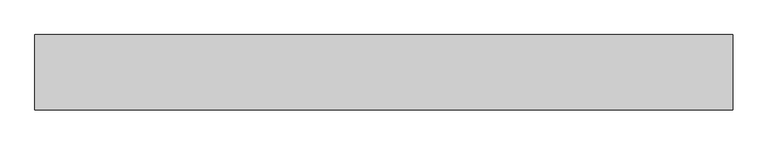
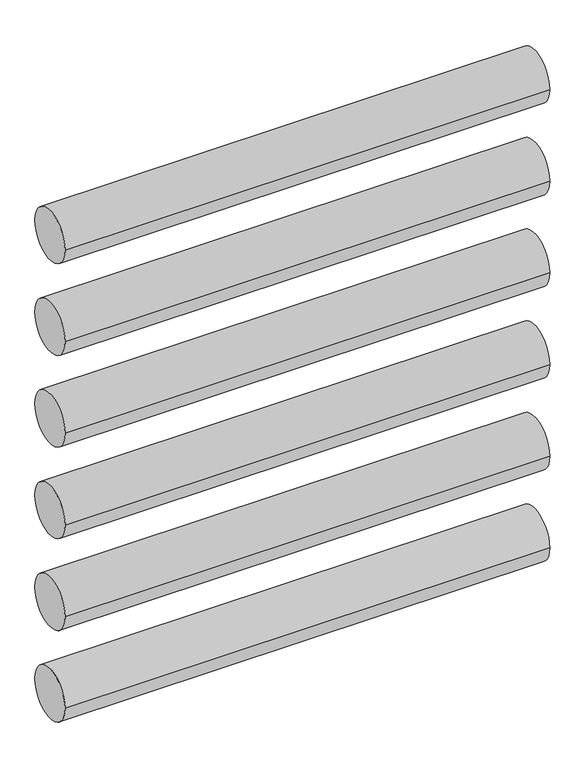
"""IFC4 building model written with IfcOpenShell, lengths in millimetres: proxy geometry, Газпремиум_Регистр : РГТ-1-108х3-1м-6."""

import ifcopenshell
import ifcopenshell.guid

model = None  # the IFC model being written
_history = None  # IfcOwnerHistory: only IFC2X3 demands one
_inside = {}  # id of a spatial element -> (the spatial element, [elements in it])
_under = {}  # id of a project, library or spatial element -> (it, [spatial elements below it])
_declared = {}  # id of a project -> (the project, [libraries it declares])
_typed = {}  # id of a type object -> (the type object, [elements of that type])
_made_of = {}  # id of a material, layer set ... -> (it, [elements and type objects made of it])


def new_model(schema):
    """Start an empty IFC model of exactly this schema.

    Asked for "IFC4X3", IfcOpenShell would pick the latest addendum, in which some entities
    have other attributes; the version numbers below select the first issue.
    IFC2X3 requires an IfcOwnerHistory on every rooted entity: one is made here for all.
    """
    global model, _history
    if schema == "IFC4X3":
        model = ifcopenshell.file(schema_version=(4, 3, 0, 0))
    else:
        model = ifcopenshell.file(schema=schema)
    _inside.clear()
    _under.clear()
    _declared.clear()
    _typed.clear()
    _made_of.clear()
    _history = None
    if model.schema == "IFC2X3":
        org = make("IfcOrganization", Name="unknown")
        user = make(
            "IfcPersonAndOrganization",
            ThePerson=make("IfcPerson", FamilyName="unknown"),
            TheOrganization=org,
        )
        app = make(
            "IfcApplication",
            ApplicationDeveloper=org,
            Version="unknown",
            ApplicationFullName="unknown",
            ApplicationIdentifier="unknown",
        )
        _history = make(
            "IfcOwnerHistory",
            OwningUser=user,
            OwningApplication=app,
            ChangeAction="ADDED",
            CreationDate=0,
        )
    return model


def make(cls, **values):
    """One entity of the class cls with the attributes given. An attribute that is None is left unset."""
    return model.create_entity(
        cls, **{name: value for name, value in values.items() if value is not None}
    )


def rooted(cls, **values):
    """An entity with a GlobalId (a new one), such as an element, a storey or a relation."""
    return make(cls, GlobalId=ifcopenshell.guid.new(), OwnerHistory=_history, **values)


def si_unit(unit_type, name, prefix=None):
    """IfcSIUnit, for example si_unit("LENGTHUNIT", "METRE", prefix="MILLI")."""
    return make("IfcSIUnit", UnitType=unit_type, Prefix=prefix, Name=name)


def assignment(units):
    """IfcUnitAssignment: the units of a project."""
    return None if units is None else make("IfcUnitAssignment", Units=units)


def point(xyz):
    """IfcCartesianPoint."""
    return None if xyz is None else make("IfcCartesianPoint", Coordinates=xyz)


def direction(xyz):
    """IfcDirection."""
    return None if xyz is None else make("IfcDirection", DirectionRatios=xyz)


def frame(location, z_axis=None, x_axis=None):
    """IfcAxis2Placement3D, a coordinate frame: its origin and axes. An axis left out is left unset."""
    return make(
        "IfcAxis2Placement3D",
        Location=point(location),
        Axis=direction(z_axis),
        RefDirection=direction(x_axis),
    )


def frame_2d(location, x_axis=None):
    """IfcAxis2Placement2D, a coordinate frame in the plane: its origin and x axis."""
    return make(
        "IfcAxis2Placement2D", Location=point(location), RefDirection=direction(x_axis)
    )


def origin():
    """The frame at (0, 0, 0) with its axes left unset."""
    return frame((0.0, 0.0, 0.0))


def place(relative_to, where):
    """IfcLocalPlacement: puts the frame where relative to a parent placement (None: the world)."""
    return make(
        "IfcLocalPlacement", PlacementRelTo=relative_to, RelativePlacement=where
    )


def context(
    kind, dimensions, precision=None, world=None, true_north=None, identifier=None
):
    """IfcGeometricRepresentationContext, for example the 3D "Model" context."""
    return make(
        "IfcGeometricRepresentationContext",
        ContextIdentifier=identifier,
        ContextType=kind,
        CoordinateSpaceDimension=dimensions,
        Precision=precision,
        WorldCoordinateSystem=world,
        TrueNorth=true_north,
    )


def project(units=None, contexts=None):
    """IfcProject with its units and contexts."""
    return rooted(
        "IfcProject",
        Name="project",
        RepresentationContexts=contexts,
        UnitsInContext=assignment(units),
    )


def spatial(cls, under=None, at=None, **own):
    """A site, building, storey or space (cls), placed at a placement, below another one or the project."""
    s = rooted(cls, ObjectPlacement=at, **own)
    if under is not None:
        _under.setdefault(under.id(), (under, []))[1].append(s)
    return s


def circle_curve(where, radius):
    """IfcCircle in the frame where."""
    return make("IfcCircle", Position=where, Radius=radius)


def trimmed(basis, trim1, trim2, sense, master):
    """IfcTrimmedCurve: the piece of a basis curve between two trims."""
    return make(
        "IfcTrimmedCurve",
        BasisCurve=basis,
        Trim1=trim1,
        Trim2=trim2,
        SenseAgreement=sense,
        MasterRepresentation=master,
    )


def segment(curve, same_sense, transition):
    """IfcCompositeCurveSegment."""
    return make(
        "IfcCompositeCurveSegment",
        Transition=transition,
        SameSense=same_sense,
        ParentCurve=curve,
    )


def composite_curve(segments, self_intersect=None):
    """IfcCompositeCurve: segments joined end to end."""
    return make("IfcCompositeCurve", Segments=segments, SelfIntersect=self_intersect)


def outline(outer, holes=None, kind="AREA"):
    """IfcArbitraryClosedProfileDef: a profile drawn as a closed curve; with holes, ...WithVoids."""
    if holes is None:
        return make("IfcArbitraryClosedProfileDef", ProfileType=kind, OuterCurve=outer)
    return make(
        "IfcArbitraryProfileDefWithVoids",
        ProfileType=kind,
        OuterCurve=outer,
        InnerCurves=holes,
    )


def extrude(swept, where, along, depth):
    """IfcExtrudedAreaSolid: the profile swept, set in the frame where, extruded along a direction by depth."""
    return make(
        "IfcExtrudedAreaSolid",
        SweptArea=swept,
        Position=where,
        ExtrudedDirection=direction(along),
        Depth=depth,
    )


def shape(context_of_items, identifier, shape_type, items):
    """IfcShapeRepresentation: the items that make up one representation, for example the "Body"."""
    return make(
        "IfcShapeRepresentation",
        ContextOfItems=context_of_items,
        RepresentationIdentifier=identifier,
        RepresentationType=shape_type,
        Items=items,
    )


def source(mapping_origin, context_of_items, identifier, shape_type, items):
    """IfcRepresentationMap: a shape defined once, which mapped items show again and again."""
    return make(
        "IfcRepresentationMap",
        MappingOrigin=mapping_origin,
        MappedRepresentation=shape(context_of_items, identifier, shape_type, items),
    )


def transform(
    local_origin,
    x_axis=None,
    y_axis=None,
    z_axis=None,
    scale=None,
    scale2=None,
    scale3=None,
    uniform=True,
):
    """IfcCartesianTransformationOperator3D, or its non-uniform kind. x_axis, y_axis, z_axis: its Axis1, 2, 3."""
    if uniform:
        return make(
            "IfcCartesianTransformationOperator3D",
            Axis1=direction(x_axis),
            Axis2=direction(y_axis),
            LocalOrigin=point(local_origin),
            Scale=scale,
            Axis3=direction(z_axis),
        )
    return make(
        "IfcCartesianTransformationOperator3DnonUniform",
        Axis1=direction(x_axis),
        Axis2=direction(y_axis),
        LocalOrigin=point(local_origin),
        Scale=scale,
        Axis3=direction(z_axis),
        Scale2=scale2,
        Scale3=scale3,
    )


def mapped(mapping_source, mapping_target):
    """IfcMappedItem: shows the shape of a source again, moved by a transform."""
    return make(
        "IfcMappedItem", MappingSource=mapping_source, MappingTarget=mapping_target
    )


def made_of(thing, what):
    """Note that an element or type object is made of a material, layer set ...; save() writes the relation."""
    if what is not None:
        _made_of.setdefault(what.id(), (what, []))[1].append(thing)
    return thing


def element(
    cls,
    number,
    at=None,
    inside=None,
    cuts=None,
    type_object=None,
    material=None,
    context=None,
    identifier="Body",
    shape_type=None,
    held_by="IfcProductDefinitionShape",
    body=None,
    shapes=None,
    **own,
):
    """One element of the class cls, such as IfcWall. Its Tag is "e" and its number.

    at: its placement. inside: the storey or other place that contains it. cuts: it is an
    opening in that element (IfcRelVoidsElement). A single representation is given by context,
    identifier, shape_type and body (its items); several are given by shapes. held_by: the class
    of the entity that holds the representations. save() writes the other relations.
    """
    e = rooted(cls, Tag="e%d" % number, ObjectPlacement=at, **own)
    if body is not None:
        shapes = [shape(context, identifier, shape_type, body)]
    if shapes is not None:
        e.Representation = make(held_by, Representations=shapes)
    if inside is not None:
        _inside.setdefault(inside.id(), (inside, []))[1].append(e)
    if cuts is not None:
        rooted(
            "IfcRelVoidsElement", RelatingBuildingElement=cuts, RelatedOpeningElement=e
        )
    if type_object is not None:
        _typed.setdefault(type_object.id(), (type_object, []))[1].append(e)
    return made_of(e, material)


def aggregate(whole, parts):
    """IfcRelAggregates: a whole, such as a stair, and the parts it consists of."""
    return rooted("IfcRelAggregates", RelatingObject=whole, RelatedObjects=parts)


def save(model, path):
    """Write the relations noted so far, then the file.

    IfcRelAggregates (storeys below a building ...), IfcRelContainedInSpatialStructure (elements
    in a storey), IfcRelDefinesByType, IfcRelAssociatesMaterial and IfcRelDeclares: one each for
    every whole, place, type object, material and project.
    """
    for whole, parts in _under.values():
        aggregate(whole, parts)
    for where, things in _inside.values():
        rooted(
            "IfcRelContainedInSpatialStructure",
            RelatedElements=things,
            RelatingStructure=where,
        )
    for kind, things in _typed.values():
        rooted("IfcRelDefinesByType", RelatedObjects=things, RelatingType=kind)
    for what, things in _made_of.values():
        rooted("IfcRelAssociatesMaterial", RelatedObjects=things, RelatingMaterial=what)
    for by, libraries in _declared.values():
        rooted("IfcRelDeclares", RelatingContext=by, RelatedDefinitions=libraries)
    model.write(path)


def mechanical_equipment_b9732147(model_context):
    return source(origin(), model_context, "Body", "SweptSolid", [
        extrude(outline(composite_curve([segment(trimmed(circle_curve(frame_2d((0.0, 1054.0)), 54.0), [point((-54.0, 1054.0))], [point((54.0, 1054.0))], False, "CARTESIAN"), True, "CONTINUOUS"), segment(trimmed(circle_curve(frame_2d((0.0, 1054.0)), 54.0), [point((54.0, 1054.0))], [point((-54.0, 1054.0))], False, "CARTESIAN"), True, "CONTINUOUS")], self_intersect=False)), frame((315.8280793, 0.0, 0.0), z_axis=(1.0, 0.0, 0.0), x_axis=(0.0, 1.0, 0.0)), (0.0, 0.0, 1.0), 1000.0),
        extrude(outline(composite_curve([segment(trimmed(circle_curve(frame_2d((0.0, 854.0)), 54.0), [point((-54.0, 854.0))], [point((54.0, 854.0))], False, "CARTESIAN"), True, "CONTINUOUS"), segment(trimmed(circle_curve(frame_2d((0.0, 854.0)), 54.0), [point((54.0, 854.0))], [point((-54.0, 854.0))], False, "CARTESIAN"), True, "CONTINUOUS")], self_intersect=False)), frame((315.8280793, 0.0, 0.0), z_axis=(1.0, 0.0, 0.0), x_axis=(0.0, 1.0, 0.0)), (0.0, 0.0, 1.0), 1000.0),
        extrude(outline(composite_curve([segment(trimmed(circle_curve(frame_2d((0.0, 654.0)), 54.0), [point((-54.0, 654.0))], [point((54.0, 654.0))], False, "CARTESIAN"), True, "CONTINUOUS"), segment(trimmed(circle_curve(frame_2d((0.0, 654.0)), 54.0), [point((54.0, 654.0))], [point((-54.0, 654.0))], False, "CARTESIAN"), True, "CONTINUOUS")], self_intersect=False)), frame((315.8280793, 0.0, 0.0), z_axis=(1.0, 0.0, 0.0), x_axis=(0.0, 1.0, 0.0)), (0.0, 0.0, 1.0), 1000.0),
        extrude(outline(composite_curve([segment(trimmed(circle_curve(frame_2d((0.0, 454.0)), 54.0), [point((-54.0, 454.0))], [point((54.0, 454.0))], False, "CARTESIAN"), True, "CONTINUOUS"), segment(trimmed(circle_curve(frame_2d((0.0, 454.0)), 54.0), [point((54.0, 454.0))], [point((-54.0, 454.0))], False, "CARTESIAN"), True, "CONTINUOUS")], self_intersect=False)), frame((315.8280793, 0.0, 0.0), z_axis=(1.0, 0.0, 0.0), x_axis=(0.0, 1.0, 0.0)), (0.0, 0.0, 1.0), 1000.0),
        extrude(outline(composite_curve([segment(trimmed(circle_curve(frame_2d((0.0, 254.0)), 54.0), [point((-54.0, 254.0))], [point((54.0, 254.0))], False, "CARTESIAN"), True, "CONTINUOUS"), segment(trimmed(circle_curve(frame_2d((0.0, 254.0)), 54.0), [point((54.0, 254.0))], [point((-54.0, 254.0))], False, "CARTESIAN"), True, "CONTINUOUS")], self_intersect=False)), frame((315.8280793, 0.0, 0.0), z_axis=(1.0, 0.0, 0.0), x_axis=(0.0, 1.0, 0.0)), (0.0, 0.0, 1.0), 1000.0),
        extrude(outline(composite_curve([segment(trimmed(circle_curve(frame_2d((0.0, 54.0)), 54.0), [point((-54.0, 54.0))], [point((54.0, 54.0))], False, "CARTESIAN"), True, "CONTINUOUS"), segment(trimmed(circle_curve(frame_2d((0.0, 54.0)), 54.0), [point((54.0, 54.0))], [point((-54.0, 54.0))], False, "CARTESIAN"), True, "CONTINUOUS")], self_intersect=False)), frame((315.8280793, 0.0, 0.0), z_axis=(1.0, 0.0, 0.0), x_axis=(0.0, 1.0, 0.0)), (0.0, 0.0, 1.0), 1000.0),
    ])


if __name__ == "__main__":
    model = new_model("IFC4")
    model_context = context("Model", 3, world=origin())
    ifc_project = project(units=[si_unit("LENGTHUNIT", "METRE", prefix="MILLI")], contexts=[model_context])
    site = spatial("IfcSite", under=ifc_project)
    building = spatial("IfcBuilding", under=site)
    placement = place(None, origin())
    mechanical_equipment_shape = mechanical_equipment_b9732147(model_context)
    element("IfcBuildingElementProxy", 1, Name="Газпремиум_Регистр : РГТ-1-108х3-1м-6", ObjectType="Газпремиум_Регистр : РГТ-1-108х3-1м-6", at=placement, inside=building, context=model_context, shape_type="MappedRepresentation", body=[
        mapped(mechanical_equipment_shape, transform((0.0, 0.0, 0.0), x_axis=(1.0, 0.0, 0.0), y_axis=(0.0, 1.0, 0.0), z_axis=(0.0, 0.0, 1.0))),
    ])
    save(model, "model.ifc")

# Revit data of these elements
# Type "Газпремиум_Регистр : РГТ-1-108х3-1м-6"
#   ADSK_Позиция = "389"
#   ADSK_Наименование = "Регистр однорядный из шести гладких труб 108х3 длиной 1 м, в комплекте с опорами и экраном"
#   ADSK_Марка = "РГТ-1-108х3-1м-6-ОП-О ТУ 4936-001-69441315-11"
#   ADSK_Код изделия = "205086?"
#   ADSK_Завод-изготовитель = "ООО ПКП \"ГазПремиум\", Россия, г.Саратов, ИНН 6452951387, кпп 645201001, gaz-premium@mail.ru"
#   ADSK_Единица измерения = "шт."
#   Расстояние между рядами = 200 mm
#   Радиус.регистра = 54 mm
#   Отступ.труб.подкл.от.осевой = 32.719 mm
#   Длина регистра = 1000 mm
#   Диаметр.труб.подкл. = 32 mm
#   Диаметр регистра = 108 mm
#   Высота = 1000 mm
#   ADSK_Масса = 36.77
#   ADSK_Количество = 1
#   Число рядов = 6
#   Соед.трубы = Грунтовка.красная
#   Регистр = Грунтовка.красная
#   Поддерж.арматура = Грунтовка.серая
#   Default Elevation = 0
# Element 1 (IfcBuildingElementProxy, "Газпремиум_Регистр : РГТ-1-108х3-1м-6")
#   Materials on its faces: "Грунтовка.красная"
# Materials
#   "Грунтовка.красная": class "Разное", colour RGB 255 0 0, transparency 0
#   "Грунтовка.серая": class "Разное", colour RGB 187 181 179, transparency 0
